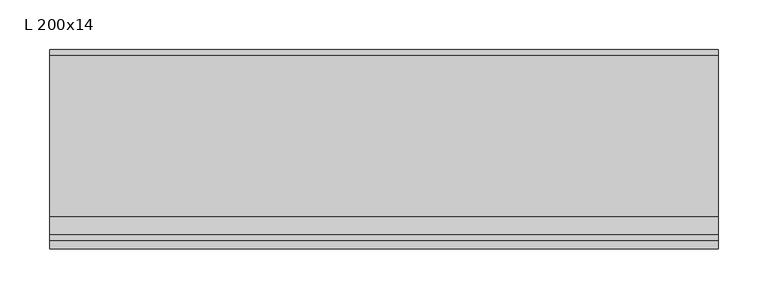
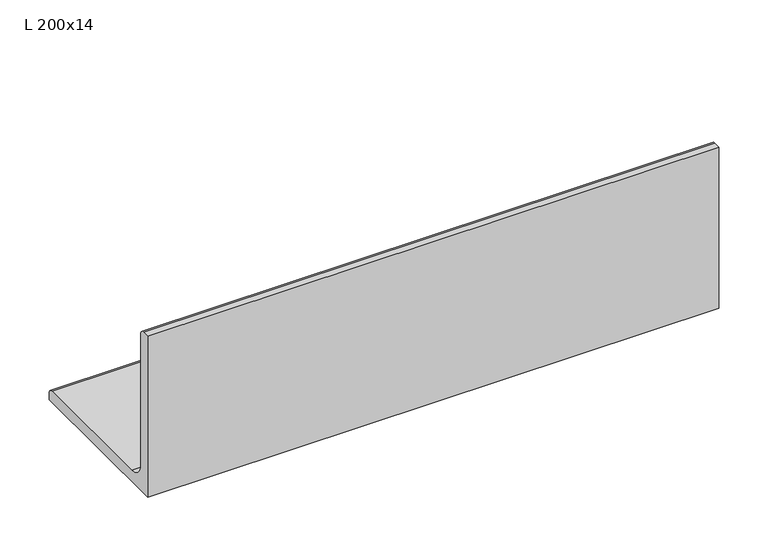
"""IFC4 building model written with IfcOpenShell, lengths in millimetres: beam geometry, Уголок (ГОСТ 8509-93) Балки : L 200x14."""

from ifc_helpers import new_model, si_unit, point, frame, frame_2d, origin, place, context, project, spatial, polyline, circle_curve, trimmed, segment, composite_curve, outline, extrude, source, transform, mapped, element, save


def l_200x14_4beb5e8d(model_context):
    return source(origin(), model_context, "Body", "SweptSolid", [
        extrude(outline(composite_curve([segment(polyline([(-54.6, -54.6), (-54.6, 145.4), (-46.6, 145.4)]), True, "CONTINUOUS"), segment(trimmed(circle_curve(frame_2d((-46.6, 139.4)), 6.0), [point((-46.6, 145.4))], [point((-40.6, 139.4))], False, "CARTESIAN"), True, "CONTINUOUS"), segment(polyline([(-40.6, 139.4), (-40.6, -22.6)]), True, "CONTINUOUS"), segment(trimmed(circle_curve(frame_2d((-22.6, -22.6)), 18.0), [point((-40.6, -22.6))], [point((-22.6, -40.6))], True, "CARTESIAN"), True, "CONTINUOUS"), segment(polyline([(-22.6, -40.6), (139.4, -40.6)]), True, "CONTINUOUS"), segment(trimmed(circle_curve(frame_2d((139.4, -46.6)), 6.0), [point((139.4, -40.6))], [point((145.4, -46.6))], False, "CARTESIAN"), True, "CONTINUOUS"), segment(polyline([(145.4, -46.6), (145.4, -54.6), (-54.6, -54.6)]), True, "CONTINUOUS")], self_intersect=False)), frame((-335.0, 0.0, 0.0), z_axis=(1.0, 0.0, 0.0), x_axis=(0.0, 1.0, 0.0)), (0.0, 0.0, 1.0), 670.0),
    ])


if __name__ == "__main__":
    model = new_model("IFC4")
    model_context = context("Model", 3, world=origin())
    ifc_project = project(units=[si_unit("LENGTHUNIT", "METRE", prefix="MILLI")], contexts=[model_context])
    site = spatial("IfcSite", under=ifc_project)
    building = spatial("IfcBuilding", under=site)
    placement = place(None, origin())
    l_200x14_shape = l_200x14_4beb5e8d(model_context)
    element("IfcBeam", 1, ObjectType="Уголок (ГОСТ 8509-93) Балки : L 200x14", at=placement, inside=building, context=model_context, shape_type="MappedRepresentation", body=[
        mapped(l_200x14_shape, transform((0.0, 0.0, 0.0), x_axis=(1.0, 0.0, 0.0), y_axis=(0.0, 1.0, 0.0), z_axis=(0.0, 0.0, 1.0))),
    ])
    save(model, "model.ifc")

# Revit data of these elements
# Type "Уголок (ГОСТ 8509-93) Балки : L 200x14"
#   ri = 6 mm
#   ra = 18 mm
#   W = 0.419725
#   Vz = 145.4 mm
#   Vy = 145.4 mm
#   Vpz = 54.6 mm
#   Vpy = 54.6 mm
#   Length [instance default] = 1500 mm
#   bf = 200 mm
#   d = 200 mm
#   tf = 14 mm
#   tw = 14 mm
#   A = 0.00546 m²
#   Structural Material [instance default] = Металл - Сталь - 345 МПa
#   Assembly Code = ""
# Element 1 (IfcBeam, "Уголок (ГОСТ 8509-93) Балки : L 200x14")
#   Structural Material = C235
#   Materials on its faces: "C235"
# Materials
#   "Металл - Сталь - 345 МПa": class "Металл", colour RGB 247 247 247, transparency 0
#   "C235": class "Не назначено", colour RGB 0 0 0, transparency 0
